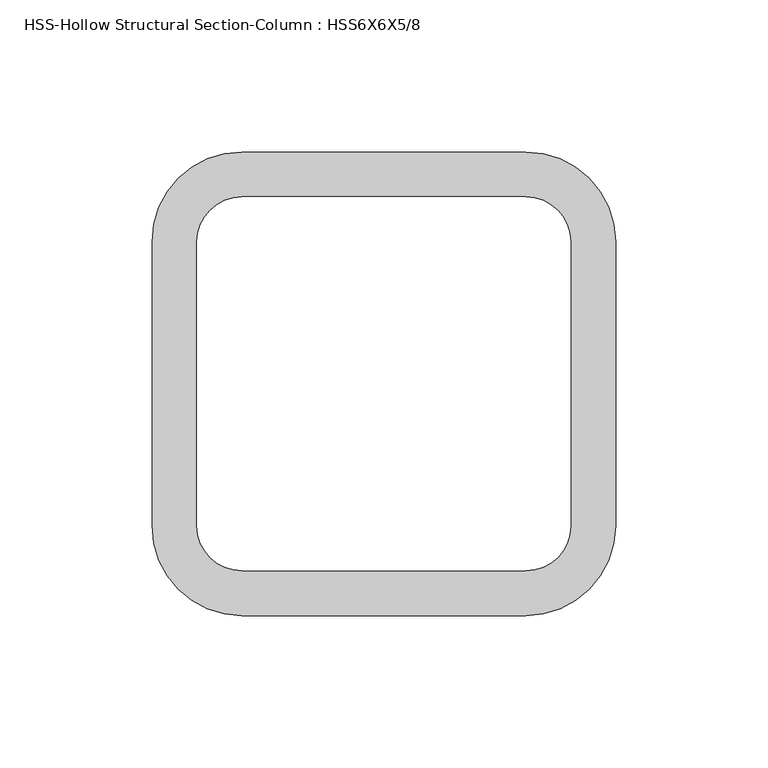
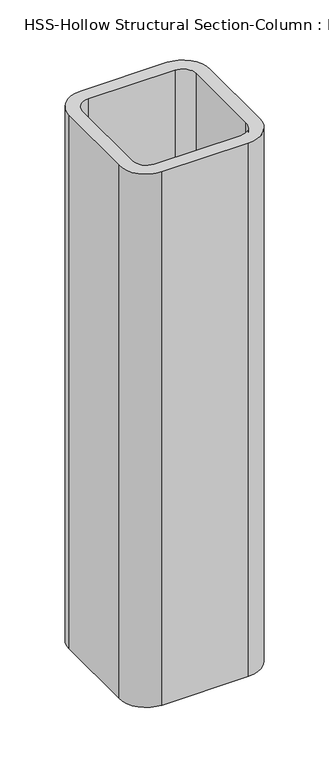
"""IFC4 building model written with IfcOpenShell, lengths in millimetres: column geometry, HSS-Hollow Structural Section-Column : HSS6X6X5/8."""

from ifc_helpers import new_model, si_unit, point, frame, frame_2d, origin, place, context, project, spatial, polyline, circle_curve, trimmed, segment, composite_curve, outline, extrude, source, transform, mapped, element, save


def hss_hollow_structural_section_column_hss6x6x5_8_cb6e0348(model_context):
    return source(origin(), model_context, "Body", "SweptSolid", [
        extrude(outline(composite_curve([segment(trimmed(circle_curve(frame_2d((46.6852, 46.6852)), 29.5148), [point((46.6852, 76.2))], [point((76.2, 46.6852))], False, "CARTESIAN"), True, "CONTINUOUS"), segment(polyline([(76.2, 46.6852), (76.2, -46.6852)]), True, "CONTINUOUS"), segment(trimmed(circle_curve(frame_2d((46.6852, -46.6852)), 29.5148), [point((76.2, -46.6852))], [point((46.6852, -76.2))], False, "CARTESIAN"), True, "CONTINUOUS"), segment(polyline([(46.6852, -76.2), (-46.6852, -76.2)]), True, "CONTINUOUS"), segment(trimmed(circle_curve(frame_2d((-46.6852, -46.6852)), 29.5148), [point((-46.6852, -76.2))], [point((-76.2, -46.6852))], False, "CARTESIAN"), True, "CONTINUOUS"), segment(polyline([(-76.2, -46.6852), (-76.2, 46.6852)]), True, "CONTINUOUS"), segment(trimmed(circle_curve(frame_2d((-46.6852, 46.6852)), 29.5148), [point((-76.2, 46.6852))], [point((-46.6852, 76.2))], False, "CARTESIAN"), True, "CONTINUOUS"), segment(polyline([(-46.6852, 76.2), (46.6852, 76.2)]), True, "CONTINUOUS")], self_intersect=False), holes=[composite_curve([segment(polyline([(46.6852, 61.4426), (-46.6852, 61.4426)]), True, "CONTINUOUS"), segment(trimmed(circle_curve(frame_2d((-46.6852, 46.6852)), 14.7574), [point((-46.6852, 61.4426))], [point((-61.4426, 46.6852))], True, "CARTESIAN"), True, "CONTINUOUS"), segment(polyline([(-61.4426, 46.6852), (-61.4426, -46.6852)]), True, "CONTINUOUS"), segment(trimmed(circle_curve(frame_2d((-46.6852, -46.6852)), 14.7574), [point((-61.4426, -46.6852))], [point((-46.6852, -61.4426))], True, "CARTESIAN"), True, "CONTINUOUS"), segment(polyline([(-46.6852, -61.4426), (46.6852, -61.4426)]), True, "CONTINUOUS"), segment(trimmed(circle_curve(frame_2d((46.6852, -46.6852)), 14.7574), [point((46.6852, -61.4426))], [point((61.4426, -46.6852))], True, "CARTESIAN"), True, "CONTINUOUS"), segment(polyline([(61.4426, -46.6852), (61.4426, 46.6852)]), True, "CONTINUOUS"), segment(trimmed(circle_curve(frame_2d((46.6852, 46.6852)), 14.7574), [point((61.4426, 46.6852))], [point((46.6852, 61.4426))], True, "CARTESIAN"), True, "CONTINUOUS")], self_intersect=False)]), frame((0.0, 0.0, -609.6), z_axis=(0.0, 0.0, 1.0), x_axis=(1.0, 0.0, 0.0)), (0.0, 0.0, 1.0), 609.6),
    ])


if __name__ == "__main__":
    model = new_model("IFC4")
    model_context = context("Model", 3, world=origin())
    ifc_project = project(units=[si_unit("LENGTHUNIT", "METRE", prefix="MILLI")], contexts=[model_context])
    site = spatial("IfcSite", under=ifc_project)
    building = spatial("IfcBuilding", under=site)
    placement = place(None, origin())
    hss_hollow_structural_section_column_hss6x6x5_8_shape = hss_hollow_structural_section_column_hss6x6x5_8_cb6e0348(model_context)
    element("IfcColumn", 1, ObjectType="HSS-Hollow Structural Section-Column : HSS6X6X5/8", at=placement, inside=building, context=model_context, shape_type="MappedRepresentation", body=[
        mapped(hss_hollow_structural_section_column_hss6x6x5_8_shape, transform((0.0, 0.0, 0.0), x_axis=(1.0, 0.0, 0.0), y_axis=(0.0, 1.0, 0.0), z_axis=(0.0, 0.0, 1.0))),
    ])
    save(model, "model.ifc")

# Revit data of these elements
# Type "HSS-Hollow Structural Section-Column : HSS6X6X5/8"
#   Assembly Code = "B10"
#   Shape = "Square"
#   W = 42.1
#   Ht = 0' - 6"
#   b = 0' - 6"
#   kr = 0' - 1.162"
#   t = 0' - 0.581"
#   A = 0.08125 SF
#   Structural Material [instance default] = Steel ASTM A500, Grade B, Rectangular and Square
# Element 1 (IfcColumn, "HSS-Hollow Structural Section-Column : HSS6X6X5/8")
#   Materials on its faces: "Steel ASTM A500, Grade B, Rectangular and Square"
# Materials
#   "Steel ASTM A500, Grade B, Rectangular and Square": class "Metal", colour RGB 199 199 199, transparency 0, Description = "Carbon steel", Cost = 0
